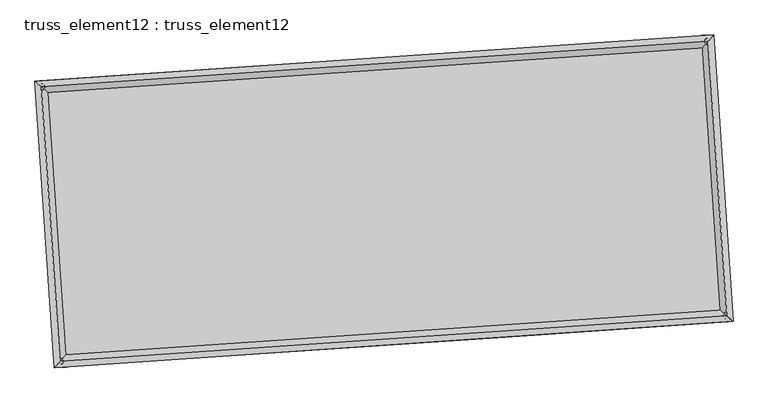
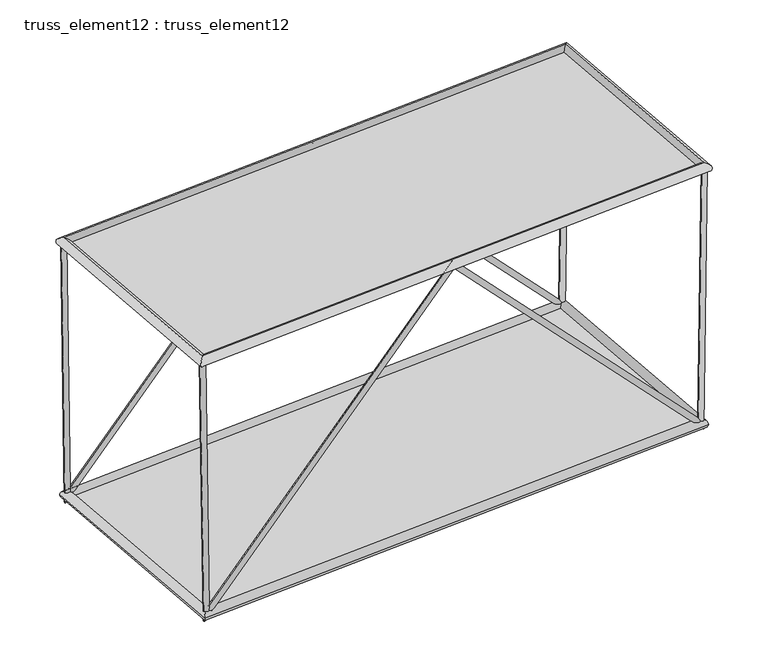
"""IFC4 building model written with IfcOpenShell, lengths in millimetres: plate geometry, truss_element12 : truss_element12."""

from ifc_helpers import new_model, si_unit, frame, origin, origin_with_axes, place, context, project, spatial, polyline, circle_curve, ellipse_curve, outline, extrude, source, transform, mapped, element, save
from ifc_brep_helpers import plane_surface, cylinder_surface, advanced_brep


def truss_element12_truss_element12_be2aad90(model_context):
    return source(origin(), model_context, "Body", "SolidModel", [
        advanced_brep(
        [(-3735.6006401, 2271.406017, 5000.2050975), (-3834.6940161, 2258.0454232, 4998.791816), (-3666.6666291, 2276.1063651, 122.4057611), (-3762.3202537, 2262.980315, -122.4057611), (1063.0860418, 2598.6102203, 5071.6275519), (1063.5437029, 2592.0376334, 4927.3870537), (5794.0749811, 2921.1983719, 122.4145359), (5890.6859959, 2921.1821166, -122.4145359), (5861.782005, 2925.8150565, 5000.2102148), (5961.7721407, 2926.0292106, 4998.822083)],
        [
            (0, 1, circle_curve(frame((-3785.1473281, 2264.7257201, 4999.4984567), z_axis=(-0.014130777343730014, -0.0009635239909554328, 0.9998996913456774), x_axis=(-0.13360615268411807, 0.9910340686191066, -0.0009331672991190194)), 50.0)),
            (1, 0, circle_curve(frame((-3785.1473281, 2264.7257201, 4999.4984567), z_axis=(-0.014130777343730014, -0.0009635239909554328, 0.9998996913456774), x_axis=(-0.13360615268411807, 0.9910340686191066, -0.0009331672991190194)), 50.0)),
            (0, 2),
            (2, 3, ellipse_curve(frame((-3714.4934414, 2269.54334, 0.0), z_axis=(-0.9284028499826127, -0.06330426115068324, 0.366143030336955), x_axis=(0.3652948219557198, 0.024908065293541812, 0.9305585856546978)), 131.8265203, 50.0)),
            (3, 1),
            (3, 2, ellipse_curve(frame((-3714.4934414, 2269.54334, 0.0), z_axis=(-0.9284028499826127, -0.06330426115068324, 0.366143030336955), x_axis=(0.3652948219557198, 0.024908065293541812, 0.9305585856546978)), 131.8265203, 50.0)),
            (2, 4),
            (4, 5, ellipse_curve(frame((1063.3148723, 2595.3239268, 4999.5073028), z_axis=(-0.9976833939203528, -0.06802823808179481, -6.571949967975178e-05), x_axis=(6.556725362871375e-05, 4.470781780485672e-06, -0.9999999978404738)), 72.2772914, 50.0)),
            (5, 3),
            (5, 4, ellipse_curve(frame((1063.3148723, 2595.3239268, 4999.5073028), z_axis=(-0.9976833939203528, -0.06802823808179481, -6.571949967975178e-05), x_axis=(6.556725362871375e-05, 4.470781780485672e-06, -0.9999999978404738)), 72.2772914, 50.0)),
            (4, 6),
            (6, 7, ellipse_curve(frame((5842.3804885, 2921.1902443, 0.0), z_axis=(-0.9283327861344512, -0.06329948376321463, -0.36632146202912796), x_axis=(-0.3654728402923341, -0.024920203687204556, 0.9304883591194691)), 131.8459204, 50.0)),
            (7, 5),
            (7, 6, ellipse_curve(frame((5842.3804885, 2921.1902443, 0.0), z_axis=(-0.9283327861344512, -0.06329948376321463, -0.36632146202912796), x_axis=(-0.3654728402923341, -0.024920203687204556, 0.9304883591194691)), 131.8459204, 50.0)),
            (8, 9, circle_curve(frame((5911.7770728, 2925.9221335, 4999.5161489), z_axis=(0.013879316866173963, 0.0009463778568815537, 0.9999032297839028), x_axis=(-0.0021544712619485026, 0.9999972590806624, -0.0009165613694543245)), 50.0)),
            (9, 8, circle_curve(frame((5911.7770728, 2925.9221335, 4999.5161489), z_axis=(0.013879316866173963, 0.0009463778568815537, 0.9999032297839028), x_axis=(-0.0021544712619485026, 0.9999972590806624, -0.0009165613694543245)), 50.0)),
            (6, 8),
            (9, 7),
        ],
        [
            plane_surface(frame((-3785.1473281, 2314.7256969, 4999.5466377), z_axis=(-0.01413077734373192, -0.0009635239909557289, 0.9998996913456774), x_axis=(0.9999001555813771, -1.3616702533525423e-05, 0.014130770783065568))),
            cylinder_surface(frame((-3785.1473281, 2264.7257201, 4999.4984567), z_axis=(-0.014130777343730014, -0.0009635239909554328, 0.9998996913456774), x_axis=(-0.13360615268411807, 0.9910340686191066, -0.0009331672991190194)), 50.0),
            cylinder_surface(frame((-3714.4934414, 2269.54334, 0.0), z_axis=(-0.6901302832567465, -0.04705736058446858, -0.7221535826586936), x_axis=(-0.020411599373552875, 0.9987523749165735, -0.04557477602268607)), 50.0),
            cylinder_surface(frame((1063.3148723, 2595.3239268, 4999.5073028), z_axis=(-0.6902249765493501, -0.04706381736012831, 0.7220626557598319), x_axis=(-0.11534328032643532, 0.9922793444614997, -0.045581029371808676)), 50.0),
            plane_surface(frame((5911.7770728, 2875.9221559, 4999.5634724), z_axis=(0.013879316866172038, 0.000946377856885389, 0.9999032297839029), x_axis=(0.999903677642666, -1.3136343474329222e-05, -0.013879310649599559))),
            cylinder_surface(frame((5842.3804885, 2921.1902443, 0.0), z_axis=(-0.013879316866173963, -0.0009463778568815537, -0.9999032297839028), x_axis=(-0.0021544712619485026, 0.9999972590806624, -0.0009165613694543245)), 50.0),
        ],
        [
            (0, [[1, 2]]),
            (1, [[-1, 3, 4, 5]]),
            (1, [[-2, -5, 6, -3]]),
            (2, [[-4, 7, 8, 9]]),
            (2, [[-6, -9, 10, -7]]),
            (3, [[-8, 11, 12, 13]]),
            (3, [[-10, -13, 14, -11]]),
            (4, [[15, 16]]),
            (5, [[-12, 17, -16, 18]]),
            (5, [[-14, -18, -15, -17]]),
        ],
    ),
        advanced_brep(
        [(-3463.4876872, -1719.3275673, 5000.2050975), (-3562.5810632, -1732.6881611, 4998.791816), (-3394.5536762, -1714.6272192, 122.4057611), (-3490.2073008, -1727.7532693, -122.4057611), (1335.1989947, -1392.123364, 5071.6275519), (1335.6566558, -1398.6959509, 4927.3870537), (6066.1879341, -1069.5352124, 122.4145359), (6162.7989488, -1069.5514677, -122.4145359), (6133.8949579, -1064.9185278, 5000.2102148), (6233.8850936, -1064.7043737, 4998.822083)],
        [
            (0, 1, circle_curve(frame((-3513.0343752, -1726.0078642, 4999.4984567), z_axis=(-0.014130777343729955, -0.000963523990955448, 0.9998996913456774), x_axis=(-0.13360615268411774, 0.9910340686191066, -0.0009331672991189919)), 50.0)),
            (1, 0, circle_curve(frame((-3513.0343752, -1726.0078642, 4999.4984567), z_axis=(-0.014130777343729955, -0.000963523990955448, 0.9998996913456774), x_axis=(-0.13360615268411774, 0.9910340686191066, -0.0009331672991189919)), 50.0)),
            (0, 2),
            (2, 3, ellipse_curve(frame((-3442.3804885, -1721.1902443, 0.0), z_axis=(-0.9284028499826127, -0.06330426115068316, 0.3661430303369552), x_axis=(0.36529482195571994, 0.024908065293541774, 0.9305585856546977)), 131.8265203, 50.0)),
            (3, 1),
            (3, 2, ellipse_curve(frame((-3442.3804885, -1721.1902443, 0.0), z_axis=(-0.9284028499826127, -0.06330426115068316, 0.3661430303369552), x_axis=(0.36529482195571994, 0.024908065293541774, 0.9305585856546977)), 131.8265203, 50.0)),
            (2, 4),
            (4, 5, ellipse_curve(frame((1335.4278253, -1395.4096575, 4999.5073028), z_axis=(-0.9976833939203528, -0.06802823808179471, -6.571949967999249e-05), x_axis=(6.556725362902129e-05, 4.470781780543329e-06, -0.9999999978404738)), 72.2772914, 50.0)),
            (5, 3),
            (5, 4, ellipse_curve(frame((1335.4278253, -1395.4096575, 4999.5073028), z_axis=(-0.9976833939203528, -0.06802823808179471, -6.571949967999249e-05), x_axis=(6.556725362902129e-05, 4.470781780543329e-06, -0.9999999978404738)), 72.2772914, 50.0)),
            (4, 6),
            (6, 7, ellipse_curve(frame((6114.4934414, -1069.54334, 0.0), z_axis=(-0.9283327861344511, -0.0632994837632146, -0.3663214620291284), x_axis=(-0.3654728402923345, -0.024920203687204566, 0.9304883591194689)), 131.8459204, 50.0)),
            (7, 5),
            (7, 6, ellipse_curve(frame((6114.4934414, -1069.54334, 0.0), z_axis=(-0.9283327861344511, -0.0632994837632146, -0.3663214620291284), x_axis=(-0.3654728402923345, -0.024920203687204566, 0.9304883591194689)), 131.8459204, 50.0)),
            (8, 9, circle_curve(frame((6183.8900257, -1064.8114508, 4999.5161489), z_axis=(0.013879316866173474, 0.0009463778568815351, 0.9999032297839028), x_axis=(-0.0021544712619487186, 0.9999972590806624, -0.000916561369454304)), 50.0)),
            (9, 8, circle_curve(frame((6183.8900257, -1064.8114508, 4999.5161489), z_axis=(0.013879316866173474, 0.0009463778568815351, 0.9999032297839028), x_axis=(-0.0021544712619487186, 0.9999972590806624, -0.000916561369454304)), 50.0)),
            (6, 8),
            (9, 7),
        ],
        [
            plane_surface(frame((-3513.0343752, -1676.0078874, 4999.5466377), z_axis=(-0.01413077734373192, -0.0009635239909557289, 0.9998996913456774), x_axis=(0.9999001555813771, -1.3616702533525423e-05, 0.014130770783065568))),
            cylinder_surface(frame((-3513.0343752, -1726.0078642, 4999.4984567), z_axis=(-0.014130777343729955, -0.000963523990955448, 0.9998996913456774), x_axis=(-0.13360615268411774, 0.9910340686191066, -0.0009331672991189919)), 50.0),
            cylinder_surface(frame((-3442.3804885, -1721.1902443, 0.0), z_axis=(-0.6901302832567464, -0.047057360584468466, -0.7221535826586933), x_axis=(-0.020411599373552827, 0.9987523749165735, -0.04557477602268599)), 50.0),
            cylinder_surface(frame((1335.4278253, -1395.4096575, 4999.5073028), z_axis=(-0.6902249765493508, -0.04706381736012834, 0.7220626557598315), x_axis=(-0.11534328032643515, 0.9922793444614998, -0.045581029371808586)), 50.0),
            plane_surface(frame((6183.8900257, -1114.8114284, 4999.5634724), z_axis=(0.013879316866172038, 0.0009463778568853864, 0.9999032297839029), x_axis=(0.999903677642666, -1.3136343474329222e-05, -0.013879310649599559))),
            cylinder_surface(frame((6114.4934414, -1069.54334, 0.0), z_axis=(-0.013879316866173474, -0.0009463778568815351, -0.9999032297839028), x_axis=(-0.0021544712619487186, 0.9999972590806624, -0.000916561369454304)), 50.0),
        ],
        [
            (0, [[1, 2]]),
            (1, [[-1, 3, 4, 5]]),
            (1, [[-2, -5, 6, -3]]),
            (2, [[-4, 7, 8, 9]]),
            (2, [[-6, -9, 10, -7]]),
            (3, [[-8, 11, 12, 13]]),
            (3, [[-10, -13, 14, -11]]),
            (4, [[15, 16]]),
            (5, [[-12, 17, -16, 18]]),
            (5, [[-14, -18, -15, -17]]),
        ],
    ),
        advanced_brep(
        [(-3513.0297394, -1726.0027261, 4909.4984569), (-3513.0390111, -1726.0130023, 5089.4984566), (-3785.1526185, 2264.7301814, 5089.4984566), (-3785.1420377, 2264.7212588, 4909.4984569), (5911.7813818, 2925.9272494, 5089.5161488), (5911.7727639, 2925.9170177, 4909.516149), (6183.8949893, -1064.8159343, 5089.5161488), (6183.8850622, -1064.8069672, 4909.516149)],
        [
            (0, 1, ellipse_curve(frame((-3513.0343752, -1726.0078642, 4999.4984567), z_axis=(-0.7535719234042865, 0.6573654662781635, -1.2871387339014257e-06), x_axis=(-0.657365466276915, -0.7535719234053757, -1.287138733901674e-06)), 127.2792206, 90.0)),
            (1, 2),
            (2, 3, ellipse_curve(frame((-3785.1473281, 2264.7257201, 4999.4984567), z_axis=(-0.657365466276915, -0.7535719234053756, -1.287138733901906e-06), x_axis=(0.7535719234042865, -0.6573654662781635, 1.2871387339016578e-06)), 127.2792206, 90.0)),
            (3, 0),
            (1, 0, ellipse_curve(frame((-3513.0343752, -1726.0078642, 4999.4984567), z_axis=(-0.7535719234042865, 0.6573654662781635, -1.2871387339014257e-06), x_axis=(-0.657365466276915, -0.7535719234053757, -1.287138733901674e-06)), 127.2792206, 90.0)),
            (3, 2, ellipse_curve(frame((-3785.1473281, 2264.7257201, 4999.4984567), z_axis=(-0.657365466276915, -0.7535719234053756, -1.287138733901906e-06), x_axis=(0.7535719234042865, -0.6573654662781635, 1.2871387339016578e-06)), 127.2792206, 90.0)),
            (2, 4),
            (4, 5, ellipse_curve(frame((5911.7770728, 2925.9221335, 4999.5161489), z_axis=(-0.7535719234042866, 0.6573654662781635, -1.2871387339018918e-06), x_axis=(-0.657365466276915, -0.7535719234053757, -1.2871387339016724e-06)), 127.2792206, 90.0)),
            (5, 3),
            (5, 4, ellipse_curve(frame((5911.7770728, 2925.9221335, 4999.5161489), z_axis=(-0.7535719234042866, 0.6573654662781635, -1.2871387339018918e-06), x_axis=(-0.657365466276915, -0.7535719234053757, -1.2871387339016724e-06)), 127.2792206, 90.0)),
            (4, 6),
            (6, 7, ellipse_curve(frame((6183.8900257, -1064.8114508, 4999.5161489), z_axis=(0.6573654662769151, 0.7535719234053756, 1.2871387339014406e-06), x_axis=(-0.7535719234042866, 0.6573654662781636, -1.2871387339016595e-06)), 127.2792206, 90.0)),
            (7, 5),
            (7, 6, ellipse_curve(frame((6183.8900257, -1064.8114508, 4999.5161489), z_axis=(0.6573654662769151, 0.7535719234053756, 1.2871387339014406e-06), x_axis=(-0.7535719234042866, 0.6573654662781636, -1.2871387339016595e-06)), 127.2792206, 90.0)),
            (6, 1),
            (0, 7),
        ],
        [
            cylinder_surface(frame((-3513.0343752, -1726.0078642, 4999.4984567), z_axis=(0.0680282382286971, -0.9976833960748769, 0.0), x_axis=(-0.9976833945508087, -0.06802823812477667, -5.5273991684341074e-05)), 90.0),
            cylinder_surface(frame((-3785.1473281, 2264.7257201, 4999.4984567), z_axis=(-0.997683396073224, -0.06802823822858504, -1.8202890541396347e-06), x_axis=(-0.06802823803443349, 0.9976833946561565, -5.3453702632802165e-05)), 90.0),
            cylinder_surface(frame((5911.7770728, 2925.9221335, 4999.5161489), z_axis=(-0.06802823822869682, 0.997683396074877, 0.0), x_axis=(0.9976833947449603, 0.06802823813801485, -5.1633413581263256e-05)), 90.0),
            cylinder_surface(frame((6183.8900257, -1064.8114508, 4999.5161489), z_axis=(0.997683396073224, 0.06802823822858474, 1.8202890541393063e-06), x_axis=(0.06802823822858474, -0.9976833946429181, -5.345370263280218e-05)), 90.0),
        ],
        [
            (0, [[1, 2, 3, 4]]),
            (0, [[5, -4, 6, -2]]),
            (1, [[-3, 7, 8, 9]]),
            (1, [[-6, -9, 10, -7]]),
            (2, [[-8, 11, 12, 13]]),
            (2, [[-10, -13, 14, -11]]),
            (3, [[-12, 15, -1, 16]]),
            (3, [[-14, -16, -5, -15]]),
        ],
    ),
        advanced_brep(
        [(-3358.7115243, -1625.2761972, 0.0), (-3526.0494527, -1817.1042913, 0.0), (-3810.4074885, 2353.2123043, 0.0), (-3618.5793943, 2185.8743758, 0.0), (5926.0494527, 3017.1042913, 0.0), (5758.7115243, 2825.2761972, 0.0), (6210.4074885, -1153.2123043, 0.0), (6018.5793943, -985.8743758, 0.0)],
        [
            (0, 1, ellipse_curve(frame((-3442.3804885, -1721.1902443, 0.0), z_axis=(-0.7535719234054593, 0.6573654662780791, 0.0), x_axis=(-0.6573654662780791, -0.7535719234054594, 0.0)), 127.2792206, 90.0)),
            (1, 2),
            (2, 3, ellipse_curve(frame((-3714.4934414, 2269.54334, 0.0), z_axis=(-0.6573654662780791, -0.7535719234054593, 0.0), x_axis=(0.7535719234054593, -0.6573654662780793, 0.0)), 127.2792206, 90.0)),
            (3, 0),
            (1, 0, ellipse_curve(frame((-3442.3804885, -1721.1902443, 0.0), z_axis=(-0.7535719234054593, 0.6573654662780791, 0.0), x_axis=(-0.6573654662780791, -0.7535719234054594, 0.0)), 127.2792206, 90.0)),
            (3, 2, ellipse_curve(frame((-3714.4934414, 2269.54334, 0.0), z_axis=(-0.6573654662780791, -0.7535719234054593, 0.0), x_axis=(0.7535719234054593, -0.6573654662780793, 0.0)), 127.2792206, 90.0)),
            (2, 4),
            (4, 5, ellipse_curve(frame((5842.3804885, 2921.1902443, 0.0), z_axis=(-0.7535719234054593, 0.6573654662780792, 0.0), x_axis=(-0.6573654662780793, -0.7535719234054592, 0.0)), 127.2792206, 90.0)),
            (5, 3),
            (5, 4, ellipse_curve(frame((5842.3804885, 2921.1902443, 0.0), z_axis=(-0.7535719234054593, 0.6573654662780792, 0.0), x_axis=(-0.6573654662780793, -0.7535719234054592, 0.0)), 127.2792206, 90.0)),
            (4, 6),
            (6, 7, ellipse_curve(frame((6114.4934414, -1069.54334, 0.0), z_axis=(0.6573654662780793, 0.7535719234054593, 0.0), x_axis=(-0.7535719234054594, 0.6573654662780792, 0.0)), 127.2792206, 90.0)),
            (7, 5),
            (7, 6, ellipse_curve(frame((6114.4934414, -1069.54334, 0.0), z_axis=(0.6573654662780793, 0.7535719234054593, 0.0), x_axis=(-0.7535719234054594, 0.6573654662780792, 0.0)), 127.2792206, 90.0)),
            (6, 1),
            (0, 7),
        ],
        [
            cylinder_surface(frame((-3442.3804885, -1721.1902443, 0.0), z_axis=(0.06802823822870308, -0.9976833960748764, 0.0), x_axis=(-0.9976833960748764, -0.06802823822870308, 0.0)), 90.0),
            cylinder_surface(frame((-3714.4934414, 2269.54334, 0.0), z_axis=(-0.9976833960748764, -0.06802823822870367, 0.0), x_axis=(-0.06802823822870367, 0.9976833960748764, 0.0)), 90.0),
            cylinder_surface(frame((5842.3804885, 2921.1902443, 0.0), z_axis=(-0.06802823822870292, 0.9976833960748764, 0.0), x_axis=(0.9976833960748764, 0.06802823822870292, 0.0)), 90.0),
            cylinder_surface(frame((6114.4934414, -1069.54334, 0.0), z_axis=(0.9976833960748764, 0.0680282382287036, 0.0), x_axis=(0.0680282382287036, -0.9976833960748764, 0.0)), 90.0),
        ],
        [
            (0, [[1, 2, 3, 4]]),
            (0, [[5, -4, 6, -2]]),
            (1, [[-3, 7, 8, 9]]),
            (1, [[-6, -9, 10, -7]]),
            (2, [[-8, 11, 12, 13]]),
            (2, [[-10, -13, 14, -11]]),
            (3, [[-12, 15, -1, 16]]),
            (3, [[-14, -16, -5, -15]]),
        ],
    ),
        extrude(outline(polyline([(-3442.3804885, -1721.1902443), (-3714.4934414, 2269.54334), (5842.3804885, 2921.1902443), (6114.4934414, -1069.54334), (-3442.3804885, -1721.1902443)])), origin_with_axes(), (0.0, 0.0, 1.0), 20.0),
        extrude(outline(polyline([(-2000.0, 4859.7202475), (2000.0, 4859.7202475), (1999.9999999, -4859.7202475), (-2000.0000001, -4859.7202474), (-2000.0, 4859.7202475)])), frame((1199.3713488, 599.9571347, 4999.5073028), z_axis=(-1.816072165371791e-06, -1.2383105742010014e-07, 0.9999999999983433), x_axis=(-0.06802823822870292, 0.9976833960748764, 0.0)), (0.0, 0.0, 1.0), 20.0),
    ])


if __name__ == "__main__":
    model = new_model("IFC4")
    model_context = context("Model", 3, world=origin())
    ifc_project = project(units=[si_unit("LENGTHUNIT", "METRE", prefix="MILLI")], contexts=[model_context])
    site = spatial("IfcSite", under=ifc_project)
    building = spatial("IfcBuilding", under=site)
    placement = place(None, origin())
    truss_element12_truss_element12_shape = truss_element12_truss_element12_be2aad90(model_context)
    element("IfcPlate", 1, ObjectType="truss_element12 : truss_element12", at=placement, inside=building, context=model_context, shape_type="MappedRepresentation", body=[
        mapped(truss_element12_truss_element12_shape, transform((0.0, 0.0, 0.0), x_axis=(1.0, 0.0, 0.0), y_axis=(0.0, 1.0, 0.0), z_axis=(0.0, 0.0, 1.0))),
    ])
    save(model, "model.ifc")

# Revit data of these elements
# Type "truss_element12 : truss_element12"
#   steellbar1 = 90 mm
#   steelbar2 = 50 mm
#   offset1 = 5000 mm
#   M = Default Roof
# Element 1 (IfcPlate, "truss_element12 : truss_element12")
#   Materials on its faces: "Default Roof"
# Materials
#   "Default Roof": class "Miscellaneous", colour RGB 0 127 0, transparency 0, Comments = "Rendering appearance not upgraded Rendering appearance not upgraded ", Cost = 0
